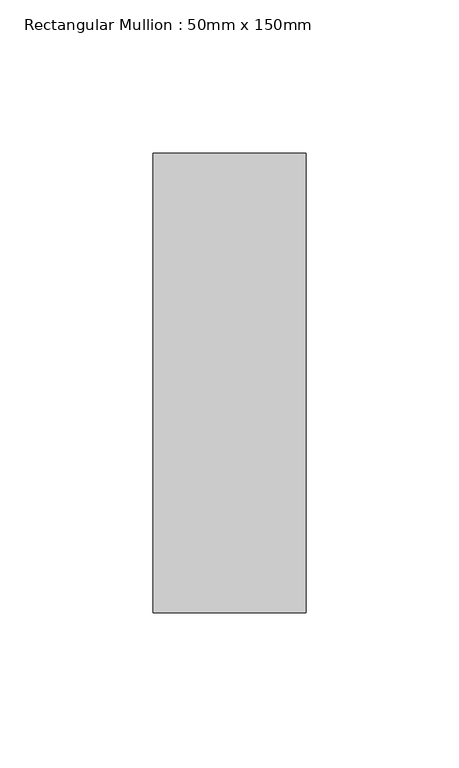
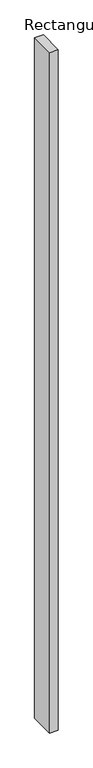
"""IFC4 building model written with IfcOpenShell, lengths in millimetres: member geometry, Rectangular Mullion : 50mm x 150mm."""

from ifc_helpers import new_model, si_unit, frame, origin, place, context, project, spatial, polyline, outline, extrude, source, transform, mapped, element, save


def rectangular_mullion_50mm_x_150mm_83adb32a(model_context):
    return source(origin(), model_context, "Body", "SweptSolid", [
        extrude(outline(polyline([(0.0, 75.0), (0.0, -75.0), (-50.0, -75.0), (-50.0, 75.0), (0.0, 75.0)])), frame((0.0, 0.0, -4165.9090909), z_axis=(0.0, 0.0, 1.0), x_axis=(1.0, 0.0, 0.0)), (0.0, 0.0, 1.0), 4165.9090909),
    ])


if __name__ == "__main__":
    model = new_model("IFC4")
    model_context = context("Model", 3, world=origin())
    ifc_project = project(units=[si_unit("LENGTHUNIT", "METRE", prefix="MILLI")], contexts=[model_context])
    site = spatial("IfcSite", under=ifc_project)
    building = spatial("IfcBuilding", under=site)
    placement = place(None, origin())
    rectangular_mullion_50mm_x_150mm_shape = rectangular_mullion_50mm_x_150mm_83adb32a(model_context)
    element("IfcMember", 1, ObjectType="Rectangular Mullion : 50mm x 150mm", at=placement, inside=building, context=model_context, shape_type="MappedRepresentation", body=[
        mapped(rectangular_mullion_50mm_x_150mm_shape, transform((0.0, 0.0, 0.0), x_axis=(1.0, 0.0, 0.0), y_axis=(0.0, 1.0, 0.0), z_axis=(0.0, 0.0, 1.0))),
    ])
    save(model, "model.ifc")

# Revit data of these elements
# Type "Rectangular Mullion : 50mm x 150mm"
#   built-in parameter 1007304 = 0.492126 (stored number, unit not read)
#   built-in parameter 1007301 = 0.082021 (stored number, unit not read)
#   built-in parameter 1007300 = 0.082021 (stored number, unit not read)
# Element 1 (IfcMember, "Rectangular Mullion : 50mm x 150mm")
#   Materials on its faces: "Aluminum"
# Materials
#   "Aluminum": class "Metal", colour RGB 244 244 244, transparency 0, Description = "Aluminum 6061", Cost = 0
